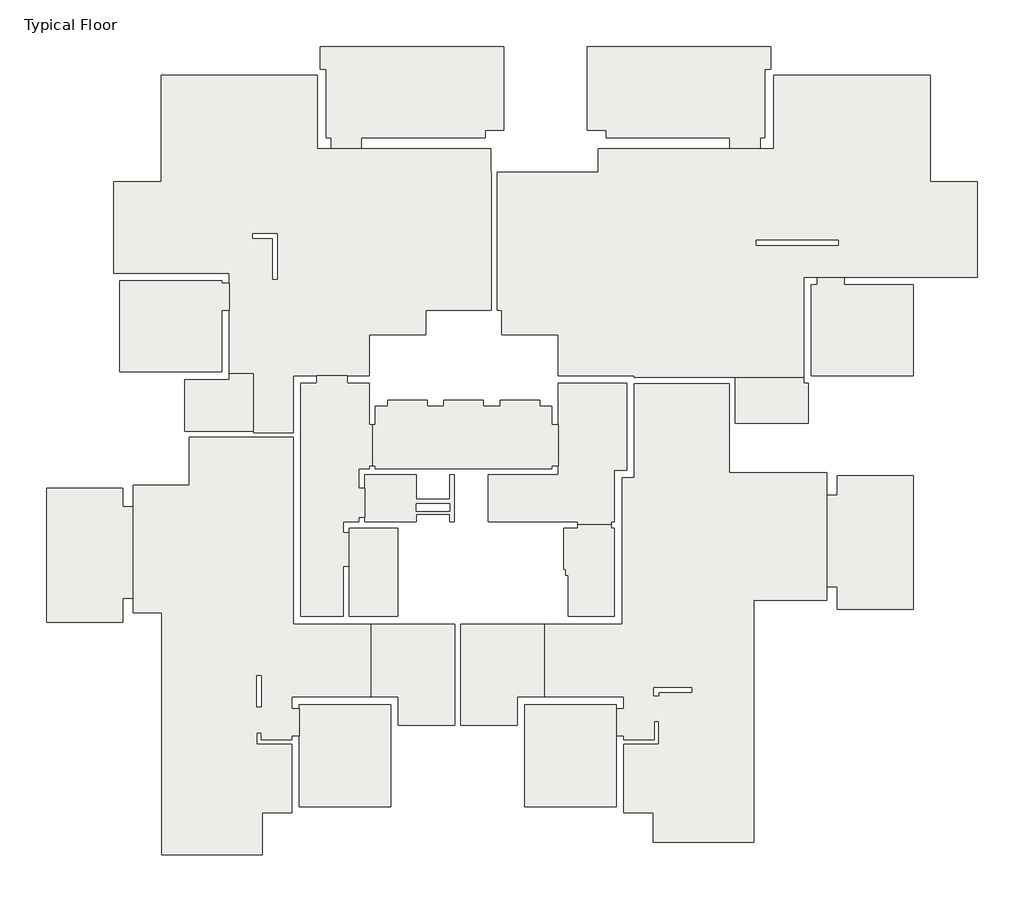
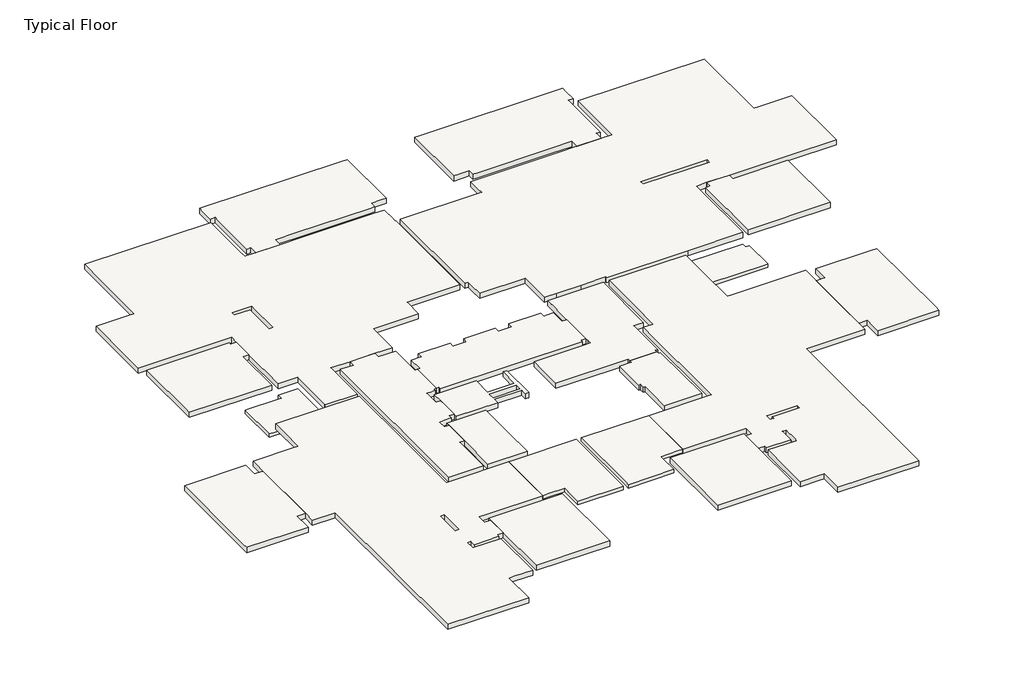
# One storey: 22 slabs.
# Revit data of these elements (continued)
# Element 14 (IfcSlab, "22") (continued)
#   Height Offset From Level = -15 cm
#   built-in parameter 1001954 = 1
#   SOFiSTiK_AMG_Scheduled = yes
#   SOFiSTiK_AMG_Adjusted = yes
#   Phase Created = New Construction
#   Materials on its faces: "Concrete"
# Element 15 (IfcSlab, "22")
#   Mark = "S11"
#   SOFiSTiK_AMG_Comments = ""
#   built-in parameter 1001955 = -1.5708 (stored number, unit not read)
#   Height Offset From Level = -15 cm
#   built-in parameter 1001954 = 1
#   SOFiSTiK_AMG_Scheduled = yes
#   SOFiSTiK_AMG_Adjusted = yes
#   Phase Created = New Construction
#   Materials on its faces: "Concrete"
# Element 16 (IfcSlab, "22")
#   Mark = "S12"
#   SOFiSTiK_AMG_Comments = ""
#   built-in parameter 1001955 = -1.5708 (stored number, unit not read)
#   Height Offset From Level = -15 cm
#   built-in parameter 1001954 = 1
#   SOFiSTiK_AMG_Scheduled = yes
#   SOFiSTiK_AMG_Adjusted = yes
#   Phase Created = New Construction
#   Materials on its faces: "Concrete"
# Element 17 (IfcSlab, "22")
#   Mark = "S13"
#   SOFiSTiK_AMG_Comments = ""
#   built-in parameter 1001955 = 1.5708 (stored number, unit not read)
#   Height Offset From Level = -15 cm
#   built-in parameter 1001954 = 1
#   SOFiSTiK_AMG_Scheduled = yes
#   SOFiSTiK_AMG_Adjusted = yes
#   Phase Created = New Construction
#   Materials on its faces: "Concrete"
# Element 18 (IfcSlab, "22")
#   Mark = "S14"
#   SOFiSTiK_AMG_Comments = ""
#   built-in parameter 1001955 = 1.5708 (stored number, unit not read)
#   Height Offset From Level = -15 cm
#   built-in parameter 1001954 = 1
#   SOFiSTiK_AMG_Scheduled = yes
#   SOFiSTiK_AMG_Adjusted = yes
#   Phase Created = New Construction
#   Materials on its faces: "Concrete"
# Element 19 (IfcSlab, "22")
#   Mark = "S15"
#   SOFiSTiK_AMG_Comments = ""
#   Height Offset From Level = -15 cm
#   built-in parameter 1001954 = 1
#   SOFiSTiK_AMG_Scheduled = yes
#   SOFiSTiK_AMG_Adjusted = yes
#   Phase Created = New Construction
#   Materials on its faces: "Concrete"
# Element 20 (IfcSlab, "22")
#   Mark = "S16"
#   SOFiSTiK_AMG_Comments = ""
#   Height Offset From Level = -15 cm
#   built-in parameter 1001954 = 1
#   SOFiSTiK_AMG_Scheduled = yes
#   SOFiSTiK_AMG_Adjusted = yes
#   Phase Created = New Construction
#   Materials on its faces: "Concrete"
# Element 21 (IfcSlab, "22")
#   Mark = "S17"
#   SOFiSTiK_AMG_Comments = ""
#   built-in parameter 1001955 = -1.5708 (stored number, unit not read)
#   Height Offset From Level = -15 cm
#   built-in parameter 1001954 = 1
#   SOFiSTiK_AMG_Scheduled = yes
#   SOFiSTiK_AMG_Adjusted = yes
#   Phase Created = New Construction
#   Materials on its faces: "Concrete"
# Element 22 (IfcSlab, "22")
#   Mark = "S18"
#   SOFiSTiK_AMG_Comments = ""
#   Height Offset From Level = -15 cm
#   built-in parameter 1001954 = 1
#   SOFiSTiK_AMG_Scheduled = yes
#   SOFiSTiK_AMG_Adjusted = yes
#   Phase Created = New Construction
#   Materials on its faces: "Concrete"
# Materials
#   "Concrete": class "Concrete", colour RGB 192 192 192, transparency 0, Keynote = "01000", Description = "Cast-in-place concrete", Cost = 0
